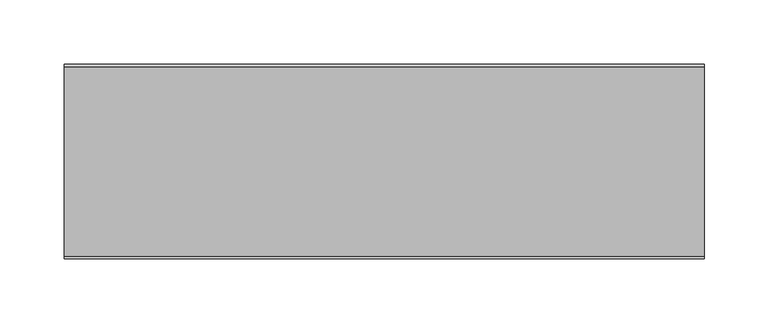
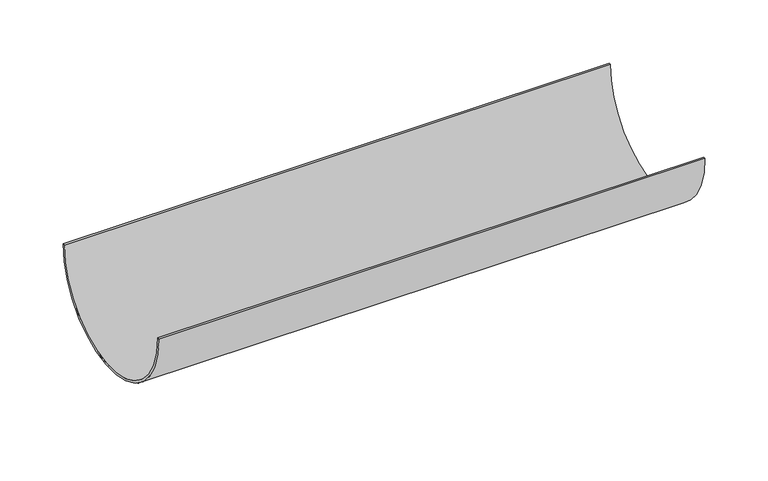
"""IFC4 building model written with IfcOpenShell, lengths in millimetres: proxy geometry, TN_ПВС 125-82_Водосточный желоб : TN_ПВС 125-82_Водосточный желоб."""

from ifc_helpers import new_model, si_unit, point, frame, origin, origin_2d, place, context, project, spatial, polyline, circle_curve, trimmed, segment, composite_curve, outline, extrude, source, transform, mapped, element, save


def generic_models_619bd3f7(model_context):
    return source(origin(), model_context, "Body", "SweptSolid", [
        extrude(outline(composite_curve([segment(trimmed(circle_curve(origin_2d(), 76.1), [point((76.1, 0.0))], [point((-76.1, 0.0))], False, "CARTESIAN"), True, "CONTINUOUS"), segment(polyline([(-76.1, 0.0), (-74.1, 0.0)]), True, "CONTINUOUS"), segment(trimmed(circle_curve(origin_2d(), 74.1), [point((-74.1, 0.0))], [point((74.1, 0.0))], True, "CARTESIAN"), True, "CONTINUOUS"), segment(polyline([(74.1, 0.0), (76.1, 0.0)]), True, "CONTINUOUS")], self_intersect=False)), frame((0.0, 0.0, 0.0), z_axis=(1.0, 0.0, 0.0), x_axis=(0.0, 1.0, 0.0)), (0.0, 0.0, 1.0), 500.0),
    ])


if __name__ == "__main__":
    model = new_model("IFC4")
    model_context = context("Model", 3, world=origin())
    ifc_project = project(units=[si_unit("LENGTHUNIT", "METRE", prefix="MILLI")], contexts=[model_context])
    site = spatial("IfcSite", under=ifc_project)
    building = spatial("IfcBuilding", under=site)
    placement = place(None, origin())
    generic_models_shape = generic_models_619bd3f7(model_context)
    element("IfcBuildingElementProxy", 1, Name="TN_ПВС 125-82_Водосточный желоб : TN_ПВС 125-82_Водосточный желоб", ObjectType="TN_ПВС 125-82_Водосточный желоб : TN_ПВС 125-82_Водосточный желоб", at=placement, inside=building, context=model_context, shape_type="MappedRepresentation", body=[
        mapped(generic_models_shape, transform((0.0, 0.0, 0.0), x_axis=(1.0, 0.0, 0.0), y_axis=(0.0, 1.0, 0.0), z_axis=(0.0, 0.0, 1.0))),
    ])
    save(model, "model.ifc")

# Revit data of these elements
# Type "TN_ПВС 125-82_Водосточный желоб : TN_ПВС 125-82_Водосточный желоб"
#   Description = "Предназначен для сбора дождевой\r\nи талой воды с кровли."
#   Manufacturer = "ТехноНИКОЛЬ"
#   Model = "Комплектующие к водосточным системам"
#   URL = "https://tn-vodostok.ru/catalog/pvh/"
#   ADSK_Обозначение = "ТехноНИКОЛЬ"
#   ADSK_Наименование краткое = "Желоб"
#   ADSK_Наименование = "Водосточный желоб"
#   ADSK_Масса_Текст = ""
#   ADSK_Марка = ""
#   ADSK_Код изделия = ""
#   ADSK_Завод-изготовитель = "ТехноНИКОЛЬ"
#   ADSK_Единица измерения = "п.м."
#   ADSK_Группирование = "Комплектующие к водосточным системам"
#   ADSK_URL страницы изделия = "https://tn-vodostok.ru/catalog/pvh/"
#   ADSK_URL документации изделия = "https://tn-vodostok.ru/upload/iblock/c42/c427963cb77eb5c3c51f0cfb870e9e52.pdf"
#   ADSK_Размер_Длина [instance default] = 500 mm
#   ADSK_Количество [instance default] = 0.5
#   ADSK_Материал [instance default] = TN_Пластик_Коричневый_RAL8019
#   Default Elevation = 0
# Element 1 (IfcBuildingElementProxy, "TN_ПВС 125-82_Водосточный желоб : TN_ПВС 125-82_Водосточный желоб")
#   Materials on its faces: "TN_Пластик_Коричневый_RAL8019"
# Materials
#   "TN_Пластик_Коричневый_RAL8019": class "Типовые", colour RGB 61 54 53, transparency 0, Cost = 0
